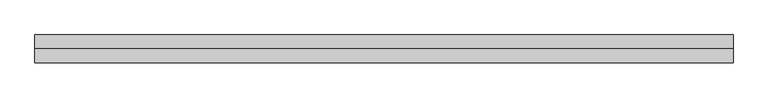
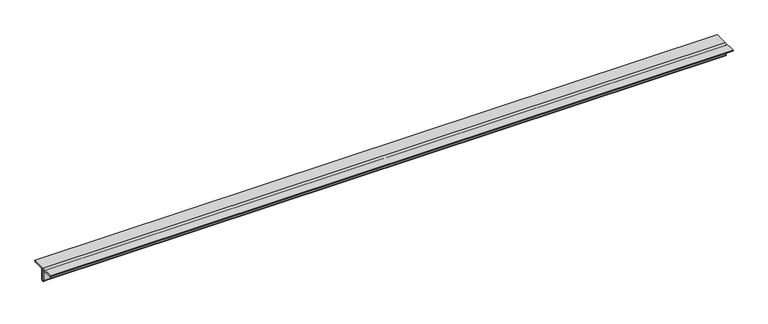
"""IFC4 building model written with IfcOpenShell, lengths in millimetres: member geometry, Steel Framing_2Ls_KS : H_SB_AR_S02_2Ls-100x100x10_VBR1."""

from ifc_helpers import new_model, si_unit, point, frame, frame_2d, origin, place, context, project, spatial, polyline, circle_curve, trimmed, segment, composite_curve, outline, extrude, source, transform, mapped, element, save


def member_95700de3(model_context):
    return source(origin(), model_context, "Body", "SweptSolid", [
        extrude(outline(composite_curve([segment(polyline([(0.0, 28.2), (0.0, -71.8)]), True, "CONTINUOUS"), segment(trimmed(circle_curve(frame_2d((0.0, -61.8)), 10.0), [point((0.0, -71.8))], [point((-10.0, -61.8))], False, "CARTESIAN"), True, "CONTINUOUS"), segment(polyline([(-10.0, -61.8), (-10.0, 8.2)]), True, "CONTINUOUS"), segment(trimmed(circle_curve(frame_2d((-20.0, 8.2)), 10.0), [point((-10.0, 8.2))], [point((-20.0, 18.2))], True, "CARTESIAN"), True, "CONTINUOUS"), segment(polyline([(-20.0, 18.2), (-90.0, 18.2)]), True, "CONTINUOUS"), segment(trimmed(circle_curve(frame_2d((-90.0, 28.2)), 10.0), [point((-90.0, 18.2))], [point((-100.0, 28.2))], False, "CARTESIAN"), True, "CONTINUOUS"), segment(polyline([(-100.0, 28.2), (0.0, 28.2)]), True, "CONTINUOUS")], self_intersect=False)), frame((-2590.3354834, 0.0, 0.0), z_axis=(1.0, 0.0, 0.0), x_axis=(0.0, 1.0, 0.0)), (0.0, 0.0, 1.0), 5034.8971694),
        extrude(outline(composite_curve([segment(polyline([(0.0, 28.2), (100.0, 28.2)]), True, "CONTINUOUS"), segment(trimmed(circle_curve(frame_2d((90.0, 28.2)), 10.0), [point((100.0, 28.2))], [point((90.0, 18.2))], False, "CARTESIAN"), True, "CONTINUOUS"), segment(polyline([(90.0, 18.2), (20.0, 18.2)]), True, "CONTINUOUS"), segment(trimmed(circle_curve(frame_2d((20.0, 8.2)), 10.0), [point((20.0, 18.2))], [point((10.0, 8.2))], True, "CARTESIAN"), True, "CONTINUOUS"), segment(polyline([(10.0, 8.2), (10.0, -61.8)]), True, "CONTINUOUS"), segment(trimmed(circle_curve(frame_2d((0.0, -61.8)), 10.0), [point((10.0, -61.8))], [point((0.0, -71.8))], False, "CARTESIAN"), True, "CONTINUOUS"), segment(polyline([(0.0, -71.8), (0.0, 28.2)]), True, "CONTINUOUS")], self_intersect=False)), frame((-2590.3354834, 0.0, 0.0), z_axis=(1.0, 0.0, 0.0), x_axis=(0.0, 1.0, 0.0)), (0.0, 0.0, 1.0), 5034.8971694),
    ])


if __name__ == "__main__":
    model = new_model("IFC4")
    model_context = context("Model", 3, world=origin())
    ifc_project = project(units=[si_unit("LENGTHUNIT", "METRE", prefix="MILLI")], contexts=[model_context])
    site = spatial("IfcSite", under=ifc_project)
    building = spatial("IfcBuilding", under=site)
    placement = place(None, origin())
    member_shape = member_95700de3(model_context)
    element("IfcMember", 1, ObjectType="Steel Framing_2Ls_KS : H_SB_AR_S02_2Ls-100x100x10_VBR1", at=placement, inside=building, context=model_context, shape_type="MappedRepresentation", body=[
        mapped(member_shape, transform((0.0, 0.0, 0.0), x_axis=(1.0, 0.0, 0.0), y_axis=(0.0, 1.0, 0.0), z_axis=(0.0, 0.0, 1.0))),
    ])
    save(model, "model.ifc")

# Revit data of these elements
# Type "Steel Framing_2Ls_KS : H_SB_AR_S02_2Ls-100x100x10_VBR1"
#   Type Comments = "MAIN"
#   Type Mark = "VBR1"
#   H_SectionID = "2Ls-100x100x10"
#   Assembly Code = "B10"
#   Legs = "LLBB"
#   H_Ratio for Additional Steel Plate = 0.2
#   W = 0
#   Perimeter = 0.80 m²/m
#   Nominal Weight = 29.80 kgf/m
#   Length [instance default] = 1524 mm
#   Space = 0 mm
#   b = 100 mm
#   d = 100 mm
#   t = 10 mm
#   y = 28.2 mm
#   A = 0.0038 m²
#   Structural Material [instance default] = Steel, 45-345
# Element 1 (IfcMember, "Steel Framing_2Ls_KS : H_SB_AR_S02_2Ls-100x100x10_VBR1")
#   Materials on its faces: "Steel, 45-345"
# Materials
#   "Steel, 45-345": class "Metal", colour RGB 189 187 185, transparency 0, Description = "Steel 345 MPa", Cost = 0
